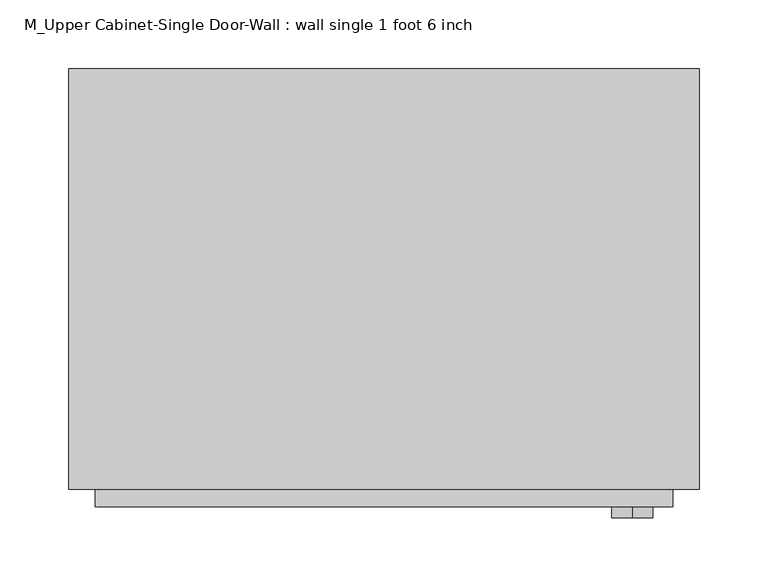
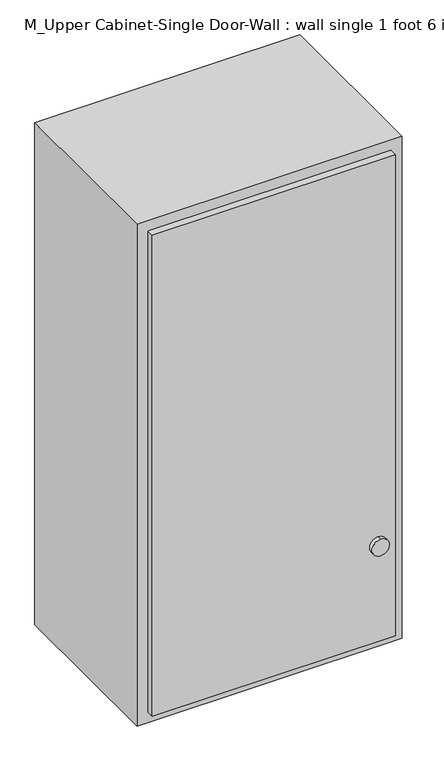
"""IFC4 building model written with IfcOpenShell, lengths in millimetres: furniture geometry, M_Upper Cabinet-Single Door-Wall : wall single 1 foot 6 inch."""

from ifc_helpers import new_model, si_unit, point, frame, frame_2d, origin, place, context, project, spatial, polyline, circle_curve, trimmed, segment, composite_curve, outline, extrude, source, transform, mapped, element, save


def m_upper_cabinet_single_door_wall_wall_single_1_foot_6_inch_8fa3af2f(model_context):
    return source(origin(), model_context, "Body", "SweptSolid", [
        extrude(outline(polyline([(-179.7788372, -373.85625), (-179.7788372, -342.10625), (239.3211628, -342.10625), (239.3211628, -373.85625), (-179.7788372, -373.85625)])), frame((0.0, 0.0, 1104.65), z_axis=(0.0, 0.0, 1.0), x_axis=(1.0, 0.0, 0.0)), (0.0, 0.0, 1.0), 876.3),
        extrude(outline(polyline([(239.3211628, -56.35625), (239.3211628, -75.40625), (-179.7788372, -75.40625), (-179.7788372, -56.35625), (239.3211628, -56.35625)])), frame((0.0, 0.0, 1104.65), z_axis=(0.0, 0.0, 1.0), x_axis=(1.0, 0.0, 0.0)), (0.0, 0.0, 1.0), 876.3),
        extrude(outline(polyline([(2000.0, -198.8288372), (1085.6, -198.8288372), (1085.6, 258.3711628), (2000.0, 258.3711628), (2000.0, -198.8288372)]), holes=[polyline([(1980.95, -179.7788372), (1980.95, 239.3211628), (1104.65, 239.3211628), (1104.65, -179.7788372), (1980.95, -179.7788372)])]), frame((0.0, -361.15625, 0.0), z_axis=(0.0, 1.0, 0.0), x_axis=(0.0, 0.0, 1.0)), (0.0, 0.0, 1.0), 304.8),
        extrude(outline(composite_curve([segment(trimmed(circle_curve(frame_2d((1280.6953371, 209.7613252)), 15.0), [point((1265.6953371, 209.7613252))], [point((1295.6953371, 209.7613252))], False, "CARTESIAN"), True, "CONTINUOUS"), segment(trimmed(circle_curve(frame_2d((1280.6953371, 209.7613252)), 15.0), [point((1295.6953371, 209.7613252))], [point((1265.6953371, 209.7613252))], False, "CARTESIAN"), True, "CONTINUOUS")], self_intersect=False)), frame((0.0, -381.85625, 0.0), z_axis=(0.0, 1.0, 0.0), x_axis=(0.0, 0.0, 1.0)), (0.0, 0.0, 1.0), 8.0),
    ])


if __name__ == "__main__":
    model = new_model("IFC4")
    model_context = context("Model", 3, world=origin())
    ifc_project = project(units=[si_unit("LENGTHUNIT", "METRE", prefix="MILLI")], contexts=[model_context])
    site = spatial("IfcSite", under=ifc_project)
    building = spatial("IfcBuilding", under=site)
    placement = place(None, origin())
    m_upper_cabinet_single_door_wall_wall_single_1_foot_6_inch_shape = m_upper_cabinet_single_door_wall_wall_single_1_foot_6_inch_8fa3af2f(model_context)
    element("IfcFurniture", 1, ObjectType="M_Upper Cabinet-Single Door-Wall : wall single 1 foot 6 inch", at=placement, inside=building, context=model_context, shape_type="MappedRepresentation", body=[
        mapped(m_upper_cabinet_single_door_wall_wall_single_1_foot_6_inch_shape, transform((0.0, 0.0, 0.0), x_axis=(1.0, 0.0, 0.0), y_axis=(0.0, 1.0, 0.0), z_axis=(0.0, 0.0, 1.0))),
    ])
    save(model, "model.ifc")

# Revit data of these elements
# Type "M_Upper Cabinet-Single Door-Wall : wall single 1 foot 6 inch"
#   Depth = 1' - 0"
#   Height = 3' - 0"
#   Top Of Cabinet = 6' - 6.74016"
#   Width = 1' - 6"
#   Cabinet Material = Base cabinet 2120100 Aspekt - 83012120100 - White
#   Door/Drawer Material = Base cabinet 2120100 Aspekt - 83012120100 - White
#   Handle Material = Cabinets - Handles
#   Default Elevation = 0
# Element 1 (IfcFurniture, "M_Upper Cabinet-Single Door-Wall : wall single 1 foot 6 inch")
#   Materials on its faces: "Base cabinet 2120100 Aspekt - 83012120100 - White"
# Materials
#   "Base cabinet 2120100 Aspekt - 83012120100 - White": class "Miscellaneous", colour RGB 255 255 255, transparency 0, Manufacturer = "Marbodal", URL = "http://www.marbodal.se", Cost = 0
#   "Cabinets - Handles": class "Metal", colour RGB 57 57 57, transparency 0
